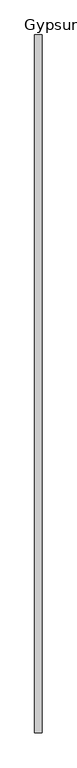
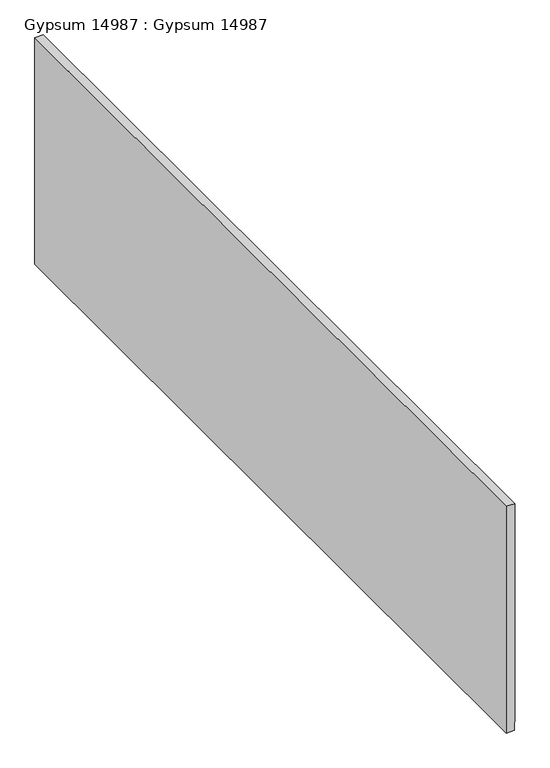
"""IFC4 building model written with IfcOpenShell, lengths in millimetres: proxy geometry, Gypsum 14987 : Gypsum 14987."""

from ifc_helpers import new_model, si_unit, frame, origin, place, context, project, spatial, polyline, outline, extrude, source, transform, mapped, element, save


def gypsum_14987_gypsum_14987_eb470674(model_context):
    return source(origin(), model_context, "Body", "SweptSolid", [
        extrude(outline(polyline([(39545.1675708, -640.491476), (39567.6883323, -640.491476), (39567.6883323, -639.211476), (40131.746, -639.211476), (40131.746, -660.156476), (39545.1675708, -660.156476), (39545.1675708, -640.491476)])), frame((0.0, -1052.8906574, 0.0), z_axis=(0.0, 1.0, 0.0), x_axis=(0.0, 0.0, 1.0)), (0.0, 0.0, 1.0), 2000.0),
    ])


if __name__ == "__main__":
    model = new_model("IFC4")
    model_context = context("Model", 3, world=origin())
    ifc_project = project(units=[si_unit("LENGTHUNIT", "METRE", prefix="MILLI")], contexts=[model_context])
    site = spatial("IfcSite", under=ifc_project)
    building = spatial("IfcBuilding", under=site)
    placement = place(None, origin())
    gypsum_14987_gypsum_14987_shape = gypsum_14987_gypsum_14987_eb470674(model_context)
    element("IfcBuildingElementProxy", 1, Name="Gypsum 14987 : Gypsum 14987", ObjectType="Gypsum 14987 : Gypsum 14987", at=placement, inside=building, context=model_context, shape_type="MappedRepresentation", body=[
        mapped(gypsum_14987_gypsum_14987_shape, transform((0.0, 0.0, 0.0), x_axis=(1.0, 0.0, 0.0), y_axis=(0.0, 1.0, 0.0), z_axis=(0.0, 0.0, 1.0))),
    ])
    save(model, "model.ifc")

# Revit data of these elements
# Type "Gypsum 14987 : Gypsum 14987"
#   NameOverride = "Gypsum"
# Element 1 (IfcBuildingElementProxy, "Gypsum 14987 : Gypsum 14987")
#   Materials on its faces: "5/8\" GYPSUM BOARD"
# Materials
#   "5/8\" GYPSUM BOARD": class "Unassigned", colour RGB 214 214 214, transparency 0, Cost = 0
